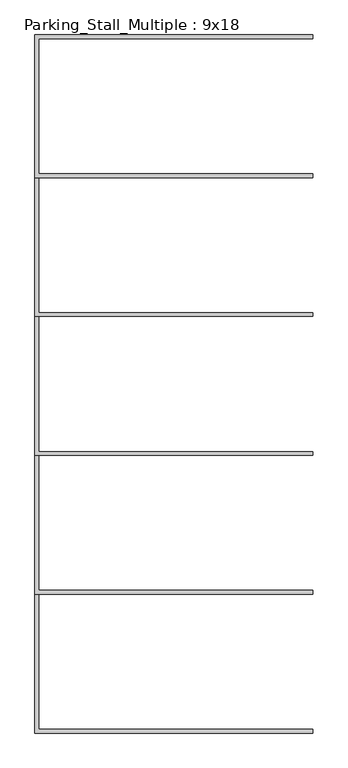
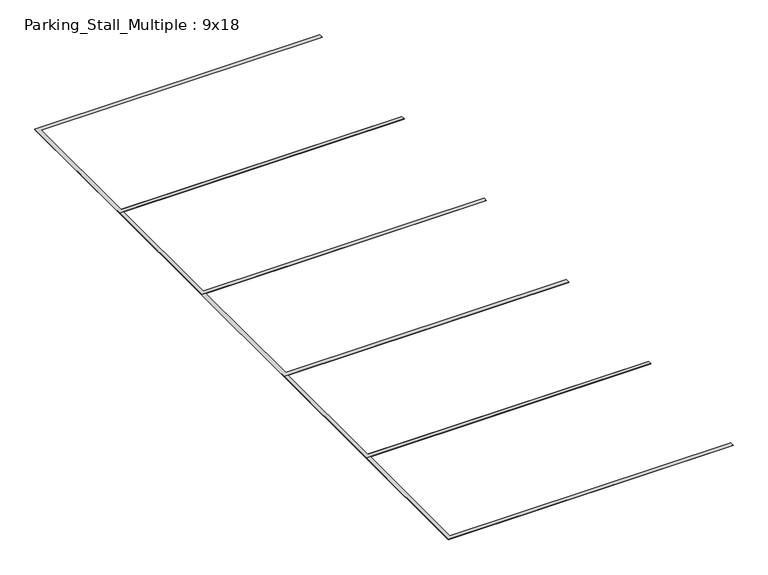
"""IFC4 building model written with IfcOpenShell, lengths in millimetres: proxy geometry, Parking_Stall_Multiple : 9x18."""

import ifcopenshell
import ifcopenshell.guid

model = None  # the IFC model being written
_history = None  # IfcOwnerHistory: only IFC2X3 demands one
_inside = {}  # id of a spatial element -> (the spatial element, [elements in it])
_under = {}  # id of a project, library or spatial element -> (it, [spatial elements below it])
_declared = {}  # id of a project -> (the project, [libraries it declares])
_typed = {}  # id of a type object -> (the type object, [elements of that type])
_made_of = {}  # id of a material, layer set ... -> (it, [elements and type objects made of it])


def new_model(schema):
    """Start an empty IFC model of exactly this schema.

    Asked for "IFC4X3", IfcOpenShell would pick the latest addendum, in which some entities
    have other attributes; the version numbers below select the first issue.
    IFC2X3 requires an IfcOwnerHistory on every rooted entity: one is made here for all.
    """
    global model, _history
    if schema == "IFC4X3":
        model = ifcopenshell.file(schema_version=(4, 3, 0, 0))
    else:
        model = ifcopenshell.file(schema=schema)
    _inside.clear()
    _under.clear()
    _declared.clear()
    _typed.clear()
    _made_of.clear()
    _history = None
    if model.schema == "IFC2X3":
        org = make("IfcOrganization", Name="unknown")
        user = make(
            "IfcPersonAndOrganization",
            ThePerson=make("IfcPerson", FamilyName="unknown"),
            TheOrganization=org,
        )
        app = make(
            "IfcApplication",
            ApplicationDeveloper=org,
            Version="unknown",
            ApplicationFullName="unknown",
            ApplicationIdentifier="unknown",
        )
        _history = make(
            "IfcOwnerHistory",
            OwningUser=user,
            OwningApplication=app,
            ChangeAction="ADDED",
            CreationDate=0,
        )
    return model


def make(cls, **values):
    """One entity of the class cls with the attributes given. An attribute that is None is left unset."""
    return model.create_entity(
        cls, **{name: value for name, value in values.items() if value is not None}
    )


def rooted(cls, **values):
    """An entity with a GlobalId (a new one), such as an element, a storey or a relation."""
    return make(cls, GlobalId=ifcopenshell.guid.new(), OwnerHistory=_history, **values)


def si_unit(unit_type, name, prefix=None):
    """IfcSIUnit, for example si_unit("LENGTHUNIT", "METRE", prefix="MILLI")."""
    return make("IfcSIUnit", UnitType=unit_type, Prefix=prefix, Name=name)


def assignment(units):
    """IfcUnitAssignment: the units of a project."""
    return None if units is None else make("IfcUnitAssignment", Units=units)


def point(xyz):
    """IfcCartesianPoint."""
    return None if xyz is None else make("IfcCartesianPoint", Coordinates=xyz)


def direction(xyz):
    """IfcDirection."""
    return None if xyz is None else make("IfcDirection", DirectionRatios=xyz)


def frame(location, z_axis=None, x_axis=None):
    """IfcAxis2Placement3D, a coordinate frame: its origin and axes. An axis left out is left unset."""
    return make(
        "IfcAxis2Placement3D",
        Location=point(location),
        Axis=direction(z_axis),
        RefDirection=direction(x_axis),
    )


def origin():
    """The frame at (0, 0, 0) with its axes left unset."""
    return frame((0.0, 0.0, 0.0))


def origin_with_axes():
    """The frame at (0, 0, 0) with the z axis (0, 0, 1) and the x axis (1, 0, 0) written out."""
    return frame((0.0, 0.0, 0.0), z_axis=(0.0, 0.0, 1.0), x_axis=(1.0, 0.0, 0.0))


def place(relative_to, where):
    """IfcLocalPlacement: puts the frame where relative to a parent placement (None: the world)."""
    return make(
        "IfcLocalPlacement", PlacementRelTo=relative_to, RelativePlacement=where
    )


def context(
    kind, dimensions, precision=None, world=None, true_north=None, identifier=None
):
    """IfcGeometricRepresentationContext, for example the 3D "Model" context."""
    return make(
        "IfcGeometricRepresentationContext",
        ContextIdentifier=identifier,
        ContextType=kind,
        CoordinateSpaceDimension=dimensions,
        Precision=precision,
        WorldCoordinateSystem=world,
        TrueNorth=true_north,
    )


def project(units=None, contexts=None):
    """IfcProject with its units and contexts."""
    return rooted(
        "IfcProject",
        Name="project",
        RepresentationContexts=contexts,
        UnitsInContext=assignment(units),
    )


def spatial(cls, under=None, at=None, **own):
    """A site, building, storey or space (cls), placed at a placement, below another one or the project."""
    s = rooted(cls, ObjectPlacement=at, **own)
    if under is not None:
        _under.setdefault(under.id(), (under, []))[1].append(s)
    return s


def polyline(points):
    """IfcPolyline through the points."""
    return make("IfcPolyline", Points=[point(p) for p in points])


def outline(outer, holes=None, kind="AREA"):
    """IfcArbitraryClosedProfileDef: a profile drawn as a closed curve; with holes, ...WithVoids."""
    if holes is None:
        return make("IfcArbitraryClosedProfileDef", ProfileType=kind, OuterCurve=outer)
    return make(
        "IfcArbitraryProfileDefWithVoids",
        ProfileType=kind,
        OuterCurve=outer,
        InnerCurves=holes,
    )


def extrude(swept, where, along, depth):
    """IfcExtrudedAreaSolid: the profile swept, set in the frame where, extruded along a direction by depth."""
    return make(
        "IfcExtrudedAreaSolid",
        SweptArea=swept,
        Position=where,
        ExtrudedDirection=direction(along),
        Depth=depth,
    )


def shape(context_of_items, identifier, shape_type, items):
    """IfcShapeRepresentation: the items that make up one representation, for example the "Body"."""
    return make(
        "IfcShapeRepresentation",
        ContextOfItems=context_of_items,
        RepresentationIdentifier=identifier,
        RepresentationType=shape_type,
        Items=items,
    )


def source(mapping_origin, context_of_items, identifier, shape_type, items):
    """IfcRepresentationMap: a shape defined once, which mapped items show again and again."""
    return make(
        "IfcRepresentationMap",
        MappingOrigin=mapping_origin,
        MappedRepresentation=shape(context_of_items, identifier, shape_type, items),
    )


def transform(
    local_origin,
    x_axis=None,
    y_axis=None,
    z_axis=None,
    scale=None,
    scale2=None,
    scale3=None,
    uniform=True,
):
    """IfcCartesianTransformationOperator3D, or its non-uniform kind. x_axis, y_axis, z_axis: its Axis1, 2, 3."""
    if uniform:
        return make(
            "IfcCartesianTransformationOperator3D",
            Axis1=direction(x_axis),
            Axis2=direction(y_axis),
            LocalOrigin=point(local_origin),
            Scale=scale,
            Axis3=direction(z_axis),
        )
    return make(
        "IfcCartesianTransformationOperator3DnonUniform",
        Axis1=direction(x_axis),
        Axis2=direction(y_axis),
        LocalOrigin=point(local_origin),
        Scale=scale,
        Axis3=direction(z_axis),
        Scale2=scale2,
        Scale3=scale3,
    )


def mapped(mapping_source, mapping_target):
    """IfcMappedItem: shows the shape of a source again, moved by a transform."""
    return make(
        "IfcMappedItem", MappingSource=mapping_source, MappingTarget=mapping_target
    )


def made_of(thing, what):
    """Note that an element or type object is made of a material, layer set ...; save() writes the relation."""
    if what is not None:
        _made_of.setdefault(what.id(), (what, []))[1].append(thing)
    return thing


def element(
    cls,
    number,
    at=None,
    inside=None,
    cuts=None,
    type_object=None,
    material=None,
    context=None,
    identifier="Body",
    shape_type=None,
    held_by="IfcProductDefinitionShape",
    body=None,
    shapes=None,
    **own,
):
    """One element of the class cls, such as IfcWall. Its Tag is "e" and its number.

    at: its placement. inside: the storey or other place that contains it. cuts: it is an
    opening in that element (IfcRelVoidsElement). A single representation is given by context,
    identifier, shape_type and body (its items); several are given by shapes. held_by: the class
    of the entity that holds the representations. save() writes the other relations.
    """
    e = rooted(cls, Tag="e%d" % number, ObjectPlacement=at, **own)
    if body is not None:
        shapes = [shape(context, identifier, shape_type, body)]
    if shapes is not None:
        e.Representation = make(held_by, Representations=shapes)
    if inside is not None:
        _inside.setdefault(inside.id(), (inside, []))[1].append(e)
    if cuts is not None:
        rooted(
            "IfcRelVoidsElement", RelatingBuildingElement=cuts, RelatedOpeningElement=e
        )
    if type_object is not None:
        _typed.setdefault(type_object.id(), (type_object, []))[1].append(e)
    return made_of(e, material)


def aggregate(whole, parts):
    """IfcRelAggregates: a whole, such as a stair, and the parts it consists of."""
    return rooted("IfcRelAggregates", RelatingObject=whole, RelatedObjects=parts)


def save(model, path):
    """Write the relations noted so far, then the file.

    IfcRelAggregates (storeys below a building ...), IfcRelContainedInSpatialStructure (elements
    in a storey), IfcRelDefinesByType, IfcRelAssociatesMaterial and IfcRelDeclares: one each for
    every whole, place, type object, material and project.
    """
    for whole, parts in _under.values():
        aggregate(whole, parts)
    for where, things in _inside.values():
        rooted(
            "IfcRelContainedInSpatialStructure",
            RelatedElements=things,
            RelatingStructure=where,
        )
    for kind, things in _typed.values():
        rooted("IfcRelDefinesByType", RelatedObjects=things, RelatingType=kind)
    for what, things in _made_of.values():
        rooted("IfcRelAssociatesMaterial", RelatedObjects=things, RelatingMaterial=what)
    for by, libraries in _declared.values():
        rooted("IfcRelDeclares", RelatingContext=by, RelatedDefinitions=libraries)
    model.write(path)


def parking_stall_multiple_9x18_ed2115c2(model_context):
    return source(origin(), model_context, "Body", "SweptSolid", [
        extrude(outline(polyline([(5486.4, 10972.8), (0.0, 10972.8), (0.0, 13792.2), (5486.4, 13792.2), (5486.4, 13716.0), (76.2, 13716.0), (76.2, 11049.0), (5486.4, 11049.0), (5486.4, 10972.8)])), origin_with_axes(), (0.0, 0.0, 1.0), 6.35),
        extrude(outline(polyline([(5486.4, 8229.6), (0.0, 8229.6), (0.0, 11049.0), (5486.4, 11049.0), (5486.4, 10972.8), (76.2, 10972.8), (76.2, 8305.8), (5486.4, 8305.8), (5486.4, 8229.6)])), origin_with_axes(), (0.0, 0.0, 1.0), 6.35),
        extrude(outline(polyline([(5486.4, 5486.4), (0.0, 5486.4), (0.0, 8305.8), (5486.4, 8305.8), (5486.4, 8229.6), (76.2, 8229.6), (76.2, 5562.6), (5486.4, 5562.6), (5486.4, 5486.4)])), origin_with_axes(), (0.0, 0.0, 1.0), 6.35),
        extrude(outline(polyline([(5486.4, 2743.2), (0.0, 2743.2), (0.0, 5562.6), (5486.4, 5562.6), (5486.4, 5486.4), (76.2, 5486.4), (76.2, 2819.4), (5486.4, 2819.4), (5486.4, 2743.2)])), origin_with_axes(), (0.0, 0.0, 1.0), 6.35),
        extrude(outline(polyline([(5486.4, 0.0), (0.0, 0.0), (0.0, 2819.4), (5486.4, 2819.4), (5486.4, 2743.2), (76.2, 2743.2), (76.2, 76.2), (5486.4, 76.2), (5486.4, 0.0)])), origin_with_axes(), (0.0, 0.0, 1.0), 6.35),
    ])


if __name__ == "__main__":
    model = new_model("IFC4")
    model_context = context("Model", 3, world=origin())
    ifc_project = project(units=[si_unit("LENGTHUNIT", "METRE", prefix="MILLI")], contexts=[model_context])
    site = spatial("IfcSite", under=ifc_project)
    building = spatial("IfcBuilding", under=site)
    placement = place(None, origin())
    parking_stall_multiple_9x18_shape = parking_stall_multiple_9x18_ed2115c2(model_context)
    element("IfcBuildingElementProxy", 1, Name="Parking_Stall_Multiple : 9x18", ObjectType="Parking_Stall_Multiple : 9x18", at=placement, inside=building, context=model_context, shape_type="MappedRepresentation", body=[
        mapped(parking_stall_multiple_9x18_shape, transform((0.0, 0.0, 0.0), x_axis=(1.0, 0.0, 0.0), y_axis=(0.0, 1.0, 0.0), z_axis=(0.0, 0.0, 1.0))),
    ])
    save(model, "model.ifc")

# Revit data of these elements
# Type "Parking_Stall_Multiple : 9x18"
#   Parking_Width_M = 9' - 0"
#   Parking_Run_Length [instance default] = 65' - 0"
#   Parking_Line_Width = 0' - 3"
#   Parking_Length_M = 18' - 0"
#   Single_Parking_Visibility [instance default] = no
#   Parking_ADA_Symbol = no
#   ParkingUnitsArray [instance default] = 7
#   ParkingUnits [instance default] = 7
#   Multiple_Parking_Visibility [instance default] = yes
#   Parking_Line_Material = none
# Element 1 (IfcBuildingElementProxy, "Parking_Stall_Multiple : 9x18")
#   Parking_Run_Length = 45' - 4.43699"
#   ParkingUnitsArray = 5
#   ParkingUnits = 5
